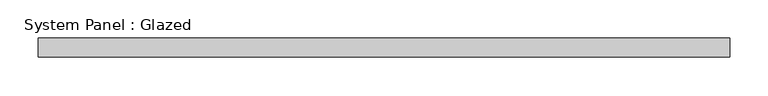
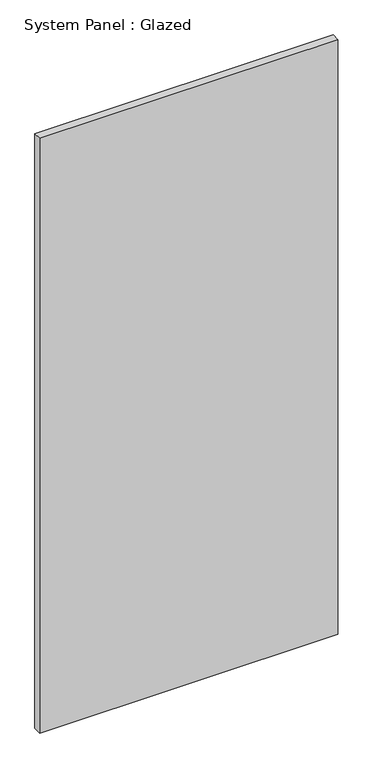
"""IFC4 building model written with IfcOpenShell, lengths in millimetres: plate geometry, System Panel : Glazed."""

from ifc_helpers import new_model, si_unit, origin, origin_with_axes, place, context, project, spatial, polyline, outline, extrude, source, transform, mapped, element, save


def system_panel_glazed_53f32d20(model_context):
    return source(origin(), model_context, "Body", "SweptSolid", [
        extrude(outline(polyline([(451.2500002, 24.5), (-451.2500002, 24.5), (-451.2500002, 49.5), (451.2500002, 49.5), (451.2500002, 24.5)])), origin_with_axes(), (0.0, 0.0, 1.0), 1902.5),
    ])


if __name__ == "__main__":
    model = new_model("IFC4")
    model_context = context("Model", 3, world=origin())
    ifc_project = project(units=[si_unit("LENGTHUNIT", "METRE", prefix="MILLI")], contexts=[model_context])
    site = spatial("IfcSite", under=ifc_project)
    building = spatial("IfcBuilding", under=site)
    placement = place(None, origin())
    system_panel_glazed_shape = system_panel_glazed_53f32d20(model_context)
    element("IfcPlate", 1, ObjectType="System Panel : Glazed", at=placement, inside=building, context=model_context, shape_type="MappedRepresentation", body=[
        mapped(system_panel_glazed_shape, transform((0.0, 0.0, 0.0), x_axis=(1.0, 0.0, 0.0), y_axis=(0.0, 1.0, 0.0), z_axis=(0.0, 0.0, 1.0))),
    ])
    save(model, "model.ifc")

# Revit data of these elements
# Type "System Panel : Glazed"
#   Construction Type Id = "GSP4R"
#   Analytic Construction = "1/8 in Pilkington single glazing"
#   Visual Light Transmittance = 0.9
#   Solar Heat Gain Coefficient = 0.86
#   Heat Transfer Coefficient (U) = 6.7069 W/(m²·K)
#   Define Thermal Properties by = 1
# Element 1 (IfcPlate, "System Panel : Glazed")
#   Materials on its faces: "Glass"
# Materials
#   "Glass": class "Glass", colour RGB 245 245 243, transparency 1, Description = "Soda Lime Glass", Cost = 0
